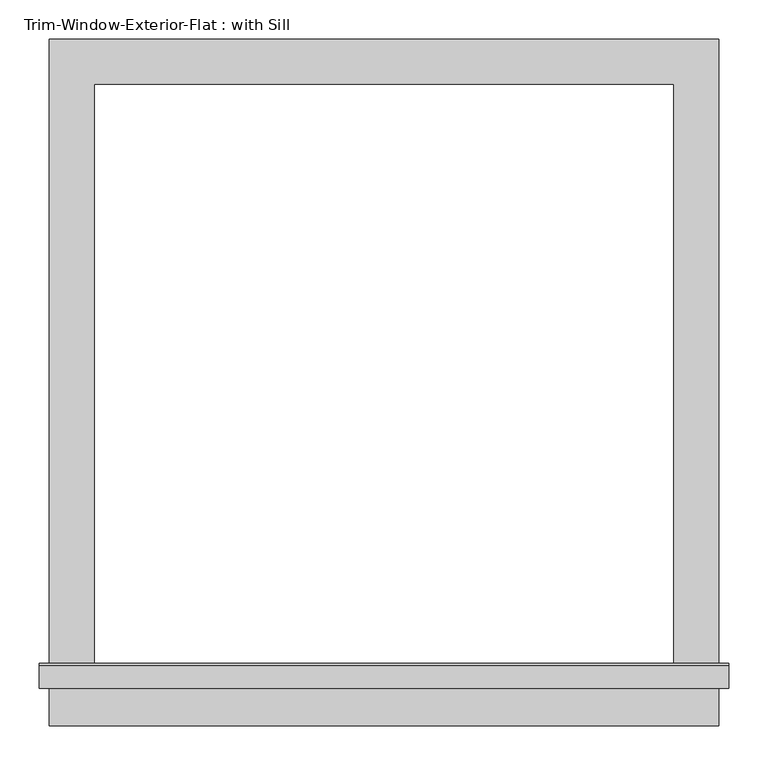
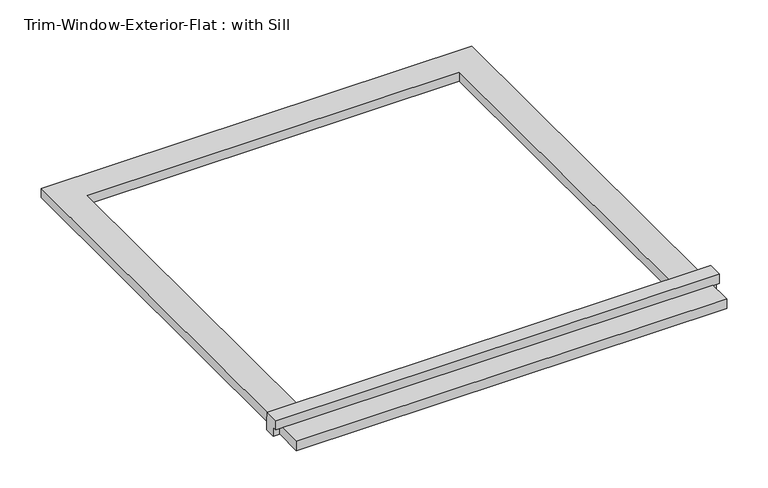
"""IFC4 building model written with IfcOpenShell, lengths in millimetres: proxy geometry, Trim-Window-Exterior-Flat : with Sill."""

from ifc_helpers import new_model, si_unit, frame, origin, origin_with_axes, place, context, project, spatial, polyline, outline, extrude, source, transform, mapped, element, save


def trim_window_exterior_flat_with_sill_b22aabc1(model_context):
    return source(origin(), model_context, "Body", "SweptSolid", [
        extrude(outline(polyline([(425.45, -758.7823709), (425.45, -815.9323709), (-425.45, -815.9323709), (-425.45, -758.7823709), (425.45, -758.7823709)])), origin_with_axes(), (0.0, 0.0, 1.0), 19.05),
        extrude(outline(polyline([(-768.35, 38.1), (-739.0580645, 38.1), (-736.6, 19.05), (-736.6, 0.0), (-758.7823709, 0.0), (-758.7823709, 19.05), (-768.35, 19.05), (-768.35, 38.1)])), frame((-438.15, 0.0, 0.0), z_axis=(1.0, 0.0, 0.0), x_axis=(0.0, 1.0, 0.0)), (0.0, 0.0, 1.0), 876.3),
        extrude(outline(polyline([(-425.45, 57.15), (425.45, 57.15), (425.45, -736.6), (368.3, -736.6), (368.3, 0.0), (-368.3, 0.0), (-368.3, -736.6), (-425.45, -736.6), (-425.45, 57.15)])), origin_with_axes(), (0.0, 0.0, 1.0), 19.05),
    ])


if __name__ == "__main__":
    model = new_model("IFC4")
    model_context = context("Model", 3, world=origin())
    ifc_project = project(units=[si_unit("LENGTHUNIT", "METRE", prefix="MILLI")], contexts=[model_context])
    site = spatial("IfcSite", under=ifc_project)
    building = spatial("IfcBuilding", under=site)
    placement = place(None, origin())
    trim_window_exterior_flat_with_sill_shape = trim_window_exterior_flat_with_sill_b22aabc1(model_context)
    element("IfcBuildingElementProxy", 1, Name="Trim-Window-Exterior-Flat : with Sill", ObjectType="Trim-Window-Exterior-Flat : with Sill", at=placement, inside=building, context=model_context, shape_type="MappedRepresentation", body=[
        mapped(trim_window_exterior_flat_with_sill_shape, transform((0.0, 0.0, 0.0), x_axis=(1.0, 0.0, 0.0), y_axis=(0.0, 1.0, 0.0), z_axis=(0.0, 0.0, 1.0))),
    ])
    save(model, "model.ifc")

# Revit data of these elements
# Type "Trim-Window-Exterior-Flat : with Sill"
#   Trim Width = 0' - 2 1/4"
#   Trim Thickness_Picture Frame = 0' - 1 1/4"
#   Trim Thickness_with Sill = 0' - 0 3/4"
#   Sill Thickness = 0' - 1 1/4"
#   Opening Width [instance default] = 2' - 0"
#   Opening Height [instance default] = 3' - 0"
#   Default Elevation = 4' - 0"
#   Sill = yes
#   Picture Frame = no
#   Trim Material [instance default] = none
# Element 1 (IfcBuildingElementProxy, "Trim-Window-Exterior-Flat : with Sill")
#   Opening Width = 2' - 5"
#   Opening Height = 2' - 5"
#   Trim Material = Clad - White
#   Materials on its faces: "Clad - White"
# Materials
#   "Clad - White": class "Wood", colour RGB 242 242 238, transparency 0, Cost = 0
